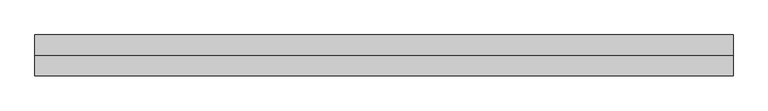
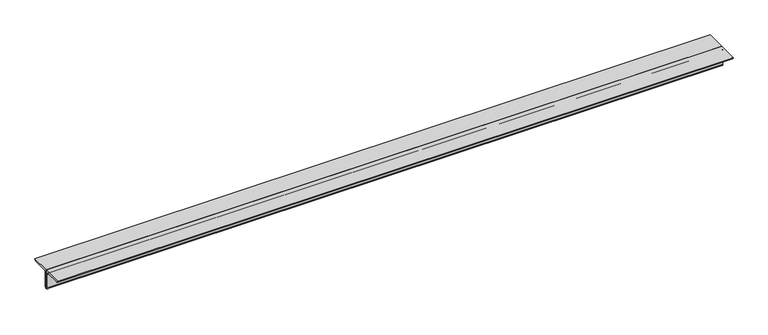
"""IFC4 building model written with IfcOpenShell, lengths in millimetres: member geometry, 0123_Steel Framing_2Ls-KSD3502 : H_SB_AR_S04_2Ls-130x130x12_VBR1."""

from ifc_helpers import new_model, si_unit, point, frame, frame_2d, origin, place, context, project, spatial, polyline, circle_curve, trimmed, segment, composite_curve, outline, extrude, source, transform, mapped, element, save


def member_1897c64a(model_context):
    return source(origin(), model_context, "Body", "SweptSolid", [
        extrude(outline(composite_curve([segment(polyline([(0.0, 36.4), (130.0, 36.4)]), True, "CONTINUOUS"), segment(trimmed(circle_curve(frame_2d((118.0, 36.4)), 12.0), [point((130.0, 36.4))], [point((118.0, 24.4))], False, "CARTESIAN"), True, "CONTINUOUS"), segment(polyline([(118.0, 24.4), (24.0, 24.4)]), True, "CONTINUOUS"), segment(trimmed(circle_curve(frame_2d((24.0, 12.4)), 12.0), [point((24.0, 24.4))], [point((12.0, 12.4))], True, "CARTESIAN"), True, "CONTINUOUS"), segment(polyline([(12.0, 12.4), (12.0, -81.6)]), True, "CONTINUOUS"), segment(trimmed(circle_curve(frame_2d((0.0, -81.6)), 12.0), [point((12.0, -81.6))], [point((0.0, -93.6))], False, "CARTESIAN"), True, "CONTINUOUS"), segment(polyline([(0.0, -93.6), (0.0, 36.4)]), True, "CONTINUOUS")], self_intersect=False)), frame((-2218.7564931, 0.0, 0.0), z_axis=(1.0, 0.0, 0.0), x_axis=(0.0, 1.0, 0.0)), (0.0, 0.0, 1.0), 4437.5129861),
        extrude(outline(composite_curve([segment(polyline([(0.0, 36.4), (0.0, -93.6)]), True, "CONTINUOUS"), segment(trimmed(circle_curve(frame_2d((0.0, -81.6)), 12.0), [point((0.0, -93.6))], [point((-12.0, -81.6))], False, "CARTESIAN"), True, "CONTINUOUS"), segment(polyline([(-12.0, -81.6), (-12.0, 12.4)]), True, "CONTINUOUS"), segment(trimmed(circle_curve(frame_2d((-24.0, 12.4)), 12.0), [point((-12.0, 12.4))], [point((-24.0, 24.4))], True, "CARTESIAN"), True, "CONTINUOUS"), segment(polyline([(-24.0, 24.4), (-118.0, 24.4)]), True, "CONTINUOUS"), segment(trimmed(circle_curve(frame_2d((-118.0, 36.4)), 12.0), [point((-118.0, 24.4))], [point((-130.0, 36.4))], False, "CARTESIAN"), True, "CONTINUOUS"), segment(polyline([(-130.0, 36.4), (0.0, 36.4)]), True, "CONTINUOUS")], self_intersect=False)), frame((-2218.7564931, 0.0, 0.0), z_axis=(1.0, 0.0, 0.0), x_axis=(0.0, 1.0, 0.0)), (0.0, 0.0, 1.0), 4437.5129861),
    ])


if __name__ == "__main__":
    model = new_model("IFC4")
    model_context = context("Model", 3, world=origin())
    ifc_project = project(units=[si_unit("LENGTHUNIT", "METRE", prefix="MILLI")], contexts=[model_context])
    site = spatial("IfcSite", under=ifc_project)
    building = spatial("IfcBuilding", under=site)
    placement = place(None, origin())
    member_shape = member_1897c64a(model_context)
    element("IfcMember", 1, ObjectType="0123_Steel Framing_2Ls-KSD3502 : H_SB_AR_S04_2Ls-130x130x12_VBR1", at=placement, inside=building, context=model_context, shape_type="MappedRepresentation", body=[
        mapped(member_shape, transform((0.0, 0.0, 0.0), x_axis=(1.0, 0.0, 0.0), y_axis=(0.0, 1.0, 0.0), z_axis=(0.0, 0.0, 1.0))),
    ])
    save(model, "model.ifc")

# Revit data of these elements
# Type "0123_Steel Framing_2Ls-KSD3502 : H_SB_AR_S04_2Ls-130x130x12_VBR1"
#   Assembly Code = "B10"
#   Legs = "SLBB"
#   W = 8.97
#   Perimeter = 1.04 m²/m
#   Nominal Weight = 46.80 kgf/m
#   Length [instance default] = 1000 mm
#   Space = 0 mm
#   b = 130 mm
#   d = 130 mm
#   t = 12 mm
#   y = 36.4 mm
#   A = 0.005952 m²
#   Structural Material [instance default] = Steel ASTM A36
# Element 1 (IfcMember, "0123_Steel Framing_2Ls-KSD3502 : H_SB_AR_S04_2Ls-130x130x12_VBR1")
#   Structural Material = Steel, 45-345
#   Materials on its faces: "Steel, 45-345"
# Materials
#   "Steel ASTM A36": class "Metal", colour RGB 199 199 199, transparency 0, Description = "Structural steel, ASTM A36 Grade B, mill finish", Cost = 0
#   "Steel, 45-345": class "Metal", colour RGB 189 187 185, transparency 0, Description = "Steel 345 MPa", Cost = 0
